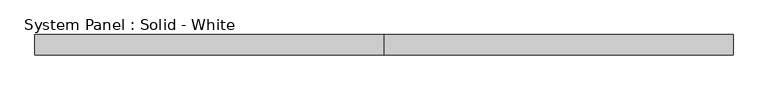
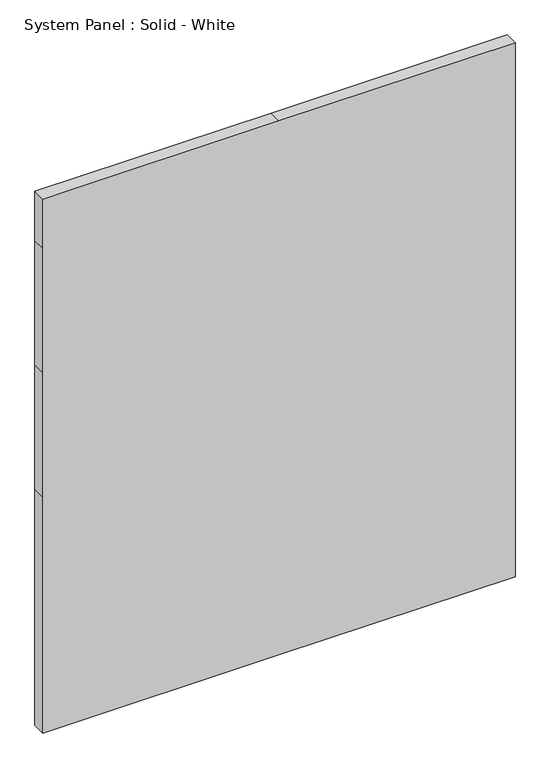
"""IFC4 building model written with IfcOpenShell, lengths in millimetres: plate geometry, System Panel : Solid - White."""

import ifcopenshell
import ifcopenshell.guid

model = None  # the IFC model being written
_history = None  # IfcOwnerHistory: only IFC2X3 demands one
_inside = {}  # id of a spatial element -> (the spatial element, [elements in it])
_under = {}  # id of a project, library or spatial element -> (it, [spatial elements below it])
_declared = {}  # id of a project -> (the project, [libraries it declares])
_typed = {}  # id of a type object -> (the type object, [elements of that type])
_made_of = {}  # id of a material, layer set ... -> (it, [elements and type objects made of it])


def new_model(schema):
    """Start an empty IFC model of exactly this schema.

    Asked for "IFC4X3", IfcOpenShell would pick the latest addendum, in which some entities
    have other attributes; the version numbers below select the first issue.
    IFC2X3 requires an IfcOwnerHistory on every rooted entity: one is made here for all.
    """
    global model, _history
    if schema == "IFC4X3":
        model = ifcopenshell.file(schema_version=(4, 3, 0, 0))
    else:
        model = ifcopenshell.file(schema=schema)
    _inside.clear()
    _under.clear()
    _declared.clear()
    _typed.clear()
    _made_of.clear()
    _history = None
    if model.schema == "IFC2X3":
        org = make("IfcOrganization", Name="unknown")
        user = make(
            "IfcPersonAndOrganization",
            ThePerson=make("IfcPerson", FamilyName="unknown"),
            TheOrganization=org,
        )
        app = make(
            "IfcApplication",
            ApplicationDeveloper=org,
            Version="unknown",
            ApplicationFullName="unknown",
            ApplicationIdentifier="unknown",
        )
        _history = make(
            "IfcOwnerHistory",
            OwningUser=user,
            OwningApplication=app,
            ChangeAction="ADDED",
            CreationDate=0,
        )
    return model


def make(cls, **values):
    """One entity of the class cls with the attributes given. An attribute that is None is left unset."""
    return model.create_entity(
        cls, **{name: value for name, value in values.items() if value is not None}
    )


def rooted(cls, **values):
    """An entity with a GlobalId (a new one), such as an element, a storey or a relation."""
    return make(cls, GlobalId=ifcopenshell.guid.new(), OwnerHistory=_history, **values)


def si_unit(unit_type, name, prefix=None):
    """IfcSIUnit, for example si_unit("LENGTHUNIT", "METRE", prefix="MILLI")."""
    return make("IfcSIUnit", UnitType=unit_type, Prefix=prefix, Name=name)


def assignment(units):
    """IfcUnitAssignment: the units of a project."""
    return None if units is None else make("IfcUnitAssignment", Units=units)


def point(xyz):
    """IfcCartesianPoint."""
    return None if xyz is None else make("IfcCartesianPoint", Coordinates=xyz)


def direction(xyz):
    """IfcDirection."""
    return None if xyz is None else make("IfcDirection", DirectionRatios=xyz)


def frame(location, z_axis=None, x_axis=None):
    """IfcAxis2Placement3D, a coordinate frame: its origin and axes. An axis left out is left unset."""
    return make(
        "IfcAxis2Placement3D",
        Location=point(location),
        Axis=direction(z_axis),
        RefDirection=direction(x_axis),
    )


def origin():
    """The frame at (0, 0, 0) with its axes left unset."""
    return frame((0.0, 0.0, 0.0))


def place(relative_to, where):
    """IfcLocalPlacement: puts the frame where relative to a parent placement (None: the world)."""
    return make(
        "IfcLocalPlacement", PlacementRelTo=relative_to, RelativePlacement=where
    )


def context(
    kind, dimensions, precision=None, world=None, true_north=None, identifier=None
):
    """IfcGeometricRepresentationContext, for example the 3D "Model" context."""
    return make(
        "IfcGeometricRepresentationContext",
        ContextIdentifier=identifier,
        ContextType=kind,
        CoordinateSpaceDimension=dimensions,
        Precision=precision,
        WorldCoordinateSystem=world,
        TrueNorth=true_north,
    )


def project(units=None, contexts=None):
    """IfcProject with its units and contexts."""
    return rooted(
        "IfcProject",
        Name="project",
        RepresentationContexts=contexts,
        UnitsInContext=assignment(units),
    )


def spatial(cls, under=None, at=None, **own):
    """A site, building, storey or space (cls), placed at a placement, below another one or the project."""
    s = rooted(cls, ObjectPlacement=at, **own)
    if under is not None:
        _under.setdefault(under.id(), (under, []))[1].append(s)
    return s


def polyline(points):
    """IfcPolyline through the points."""
    return make("IfcPolyline", Points=[point(p) for p in points])


def outline(outer, holes=None, kind="AREA"):
    """IfcArbitraryClosedProfileDef: a profile drawn as a closed curve; with holes, ...WithVoids."""
    if holes is None:
        return make("IfcArbitraryClosedProfileDef", ProfileType=kind, OuterCurve=outer)
    return make(
        "IfcArbitraryProfileDefWithVoids",
        ProfileType=kind,
        OuterCurve=outer,
        InnerCurves=holes,
    )


def extrude(swept, where, along, depth):
    """IfcExtrudedAreaSolid: the profile swept, set in the frame where, extruded along a direction by depth."""
    return make(
        "IfcExtrudedAreaSolid",
        SweptArea=swept,
        Position=where,
        ExtrudedDirection=direction(along),
        Depth=depth,
    )


def shape(context_of_items, identifier, shape_type, items):
    """IfcShapeRepresentation: the items that make up one representation, for example the "Body"."""
    return make(
        "IfcShapeRepresentation",
        ContextOfItems=context_of_items,
        RepresentationIdentifier=identifier,
        RepresentationType=shape_type,
        Items=items,
    )


def source(mapping_origin, context_of_items, identifier, shape_type, items):
    """IfcRepresentationMap: a shape defined once, which mapped items show again and again."""
    return make(
        "IfcRepresentationMap",
        MappingOrigin=mapping_origin,
        MappedRepresentation=shape(context_of_items, identifier, shape_type, items),
    )


def transform(
    local_origin,
    x_axis=None,
    y_axis=None,
    z_axis=None,
    scale=None,
    scale2=None,
    scale3=None,
    uniform=True,
):
    """IfcCartesianTransformationOperator3D, or its non-uniform kind. x_axis, y_axis, z_axis: its Axis1, 2, 3."""
    if uniform:
        return make(
            "IfcCartesianTransformationOperator3D",
            Axis1=direction(x_axis),
            Axis2=direction(y_axis),
            LocalOrigin=point(local_origin),
            Scale=scale,
            Axis3=direction(z_axis),
        )
    return make(
        "IfcCartesianTransformationOperator3DnonUniform",
        Axis1=direction(x_axis),
        Axis2=direction(y_axis),
        LocalOrigin=point(local_origin),
        Scale=scale,
        Axis3=direction(z_axis),
        Scale2=scale2,
        Scale3=scale3,
    )


def mapped(mapping_source, mapping_target):
    """IfcMappedItem: shows the shape of a source again, moved by a transform."""
    return make(
        "IfcMappedItem", MappingSource=mapping_source, MappingTarget=mapping_target
    )


def made_of(thing, what):
    """Note that an element or type object is made of a material, layer set ...; save() writes the relation."""
    if what is not None:
        _made_of.setdefault(what.id(), (what, []))[1].append(thing)
    return thing


def element(
    cls,
    number,
    at=None,
    inside=None,
    cuts=None,
    type_object=None,
    material=None,
    context=None,
    identifier="Body",
    shape_type=None,
    held_by="IfcProductDefinitionShape",
    body=None,
    shapes=None,
    **own,
):
    """One element of the class cls, such as IfcWall. Its Tag is "e" and its number.

    at: its placement. inside: the storey or other place that contains it. cuts: it is an
    opening in that element (IfcRelVoidsElement). A single representation is given by context,
    identifier, shape_type and body (its items); several are given by shapes. held_by: the class
    of the entity that holds the representations. save() writes the other relations.
    """
    e = rooted(cls, Tag="e%d" % number, ObjectPlacement=at, **own)
    if body is not None:
        shapes = [shape(context, identifier, shape_type, body)]
    if shapes is not None:
        e.Representation = make(held_by, Representations=shapes)
    if inside is not None:
        _inside.setdefault(inside.id(), (inside, []))[1].append(e)
    if cuts is not None:
        rooted(
            "IfcRelVoidsElement", RelatingBuildingElement=cuts, RelatedOpeningElement=e
        )
    if type_object is not None:
        _typed.setdefault(type_object.id(), (type_object, []))[1].append(e)
    return made_of(e, material)


def aggregate(whole, parts):
    """IfcRelAggregates: a whole, such as a stair, and the parts it consists of."""
    return rooted("IfcRelAggregates", RelatingObject=whole, RelatedObjects=parts)


def save(model, path):
    """Write the relations noted so far, then the file.

    IfcRelAggregates (storeys below a building ...), IfcRelContainedInSpatialStructure (elements
    in a storey), IfcRelDefinesByType, IfcRelAssociatesMaterial and IfcRelDeclares: one each for
    every whole, place, type object, material and project.
    """
    for whole, parts in _under.values():
        aggregate(whole, parts)
    for where, things in _inside.values():
        rooted(
            "IfcRelContainedInSpatialStructure",
            RelatedElements=things,
            RelatingStructure=where,
        )
    for kind, things in _typed.values():
        rooted("IfcRelDefinesByType", RelatedObjects=things, RelatingType=kind)
    for what, things in _made_of.values():
        rooted("IfcRelAssociatesMaterial", RelatedObjects=things, RelatingMaterial=what)
    for by, libraries in _declared.values():
        rooted("IfcRelDeclares", RelatingContext=by, RelatedDefinitions=libraries)
    model.write(path)


def system_panel_solid_white_63a197de(model_context):
    return source(origin(), model_context, "Body", "SweptSolid", [
        extrude(outline(polyline([(0.0, -1094.2054237), (0.0, 0.0), (0.0, 1094.2054237), (1155.7, 1094.2054237), (1765.3, 1094.2054237), (2374.9, 1094.2054237), (2616.2, 1094.2054237), (2616.2, 0.0), (2616.2, -1094.2054237), (2374.9, -1094.2054237), (1765.3, -1094.2054237), (1155.7, -1094.2054237), (0.0, -1094.2054237)])), frame((0.0, -44.45, 0.0), z_axis=(0.0, 1.0, 0.0), x_axis=(0.0, 0.0, 1.0)), (0.0, 0.0, 1.0), 63.5),
    ])


if __name__ == "__main__":
    model = new_model("IFC4")
    model_context = context("Model", 3, world=origin())
    ifc_project = project(units=[si_unit("LENGTHUNIT", "METRE", prefix="MILLI")], contexts=[model_context])
    site = spatial("IfcSite", under=ifc_project)
    building = spatial("IfcBuilding", under=site)
    placement = place(None, origin())
    system_panel_solid_white_shape = system_panel_solid_white_63a197de(model_context)
    element("IfcPlate", 1, ObjectType="System Panel : Solid - White", at=placement, inside=building, context=model_context, shape_type="MappedRepresentation", body=[
        mapped(system_panel_solid_white_shape, transform((0.0, 0.0, 0.0), x_axis=(1.0, 0.0, 0.0), y_axis=(0.0, 1.0, 0.0), z_axis=(0.0, 0.0, 1.0))),
    ])
    save(model, "model.ifc")

# Revit data of these elements
# Element 1 (IfcPlate, "System Panel : Solid - White")
#   Materials on its faces: "White Panel"
# Materials
#   "White Panel": class "Unassigned", colour RGB 255 255 255, transparency 0
